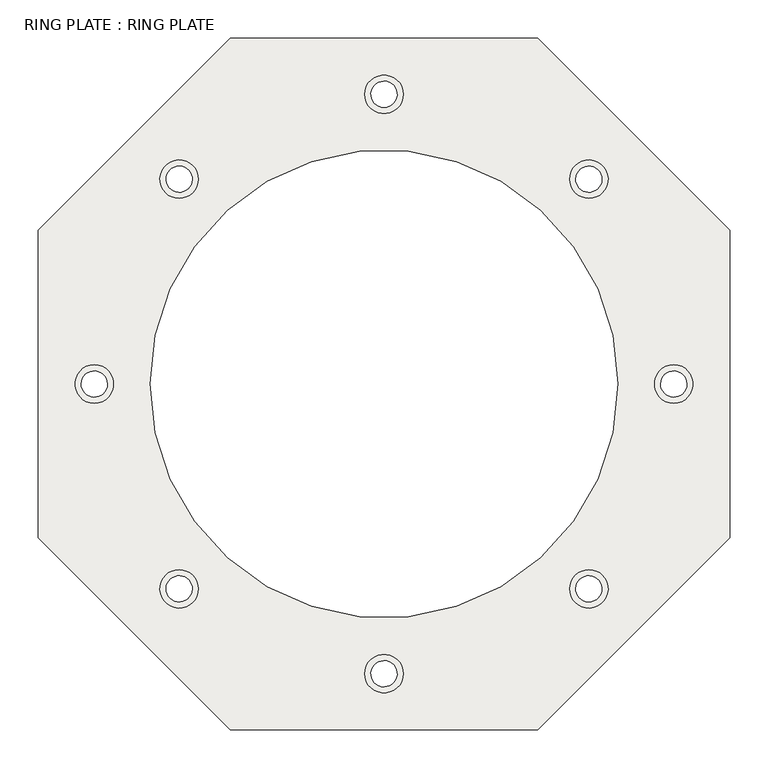
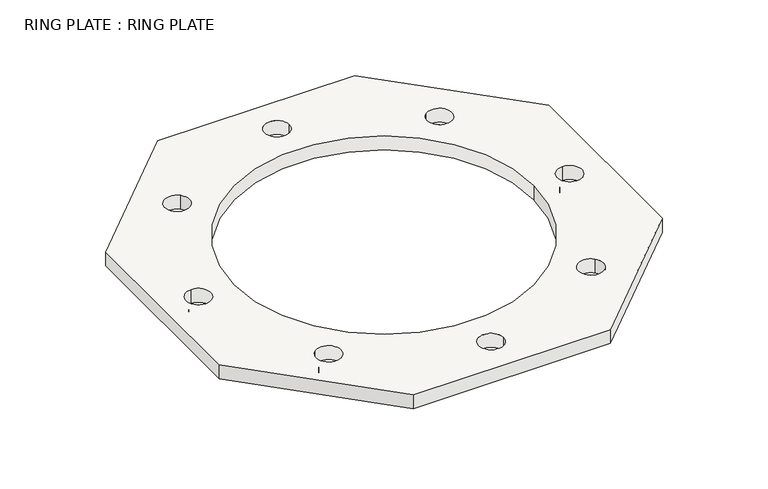
"""IFC4 building model written with IfcOpenShell, lengths in millimetres: slab geometry, RING PLATE : RING PLATE."""

from ifc_helpers import new_model, si_unit, point, frame, frame_2d, origin, place, context, project, spatial, polyline, circle_curve, trimmed, segment, composite_curve, outline, extrude, source, transform, mapped, element, save


def ring_plate_ring_plate_2bacfa3f(model_context):
    return source(origin(), model_context, "Body", "SweptSolid", [
        extrude(outline(polyline([(266.7560332, 19296.404436), (298.5758384, 19264.5846308), (316.2535079, 19246.9069613), (330.3956435, 19232.7648257), (266.7560332, 19169.1252154), (252.6138976, 19183.267351), (234.936228, 19200.9450205), (203.1164229, 19232.7648257), (266.7560332, 19296.404436)]), holes=[composite_curve([segment(trimmed(circle_curve(frame_2d((266.7560332, 19232.7648257)), 17.0), [point((266.1315996, 19215.7762977))], [point((267.3804668, 19249.7533537))], True, "CARTESIAN"), True, "CONTINUOUS"), segment(trimmed(circle_curve(frame_2d((266.7560332, 19232.7648257)), 17.0), [point((267.3804668, 19249.7533537))], [point((266.1315996, 19215.7762977))], True, "CARTESIAN"), True, "CONTINUOUS")], self_intersect=False)]), frame((0.0, 0.0, 200.0), z_axis=(0.0, 0.0, 1.0), x_axis=(1.0, 0.0, 0.0)), (0.0, 0.0, 1.0), 10.0),
        extrude(outline(polyline([(332.25, 19544.5208589), (377.25, 19544.5208589), (402.25, 19544.5208589), (422.25, 19544.5208589), (422.25, 19454.5208589), (402.25, 19454.5208589), (377.25, 19454.5208589), (332.25, 19454.5208589), (332.25, 19544.5208589)]), holes=[composite_curve([segment(trimmed(circle_curve(frame_2d((377.25, 19499.5208589)), 17.0), [point((388.8211621, 19487.0666143))], [point((365.6788379, 19511.9751035))], True, "CARTESIAN"), True, "CONTINUOUS"), segment(trimmed(circle_curve(frame_2d((377.25, 19499.5208589)), 17.0), [point((365.6788379, 19511.9751035))], [point((388.8211621, 19487.0666143))], True, "CARTESIAN"), True, "CONTINUOUS")], self_intersect=False)]), frame((0.0, 0.0, 200.0), z_axis=(0.0, 0.0, 1.0), x_axis=(1.0, 0.0, 0.0)), (0.0, 0.0, 1.0), 10.0),
        extrude(outline(polyline([(203.1164229, 19766.2768921), (234.936228, 19798.0966972), (252.6138976, 19815.7743668), (266.7560332, 19829.9165024), (330.3956435, 19766.2768921), (316.2535079, 19752.1347565), (298.5758384, 19734.4570869), (266.7560332, 19702.6372818), (203.1164229, 19766.2768921)]), holes=[composite_curve([segment(trimmed(circle_curve(frame_2d((266.7560332, 19766.2768921)), 17.0), [point((283.7445612, 19765.6524585))], [point((249.7675052, 19766.9013257))], True, "CARTESIAN"), True, "CONTINUOUS"), segment(trimmed(circle_curve(frame_2d((266.7560332, 19766.2768921)), 17.0), [point((249.7675052, 19766.9013257))], [point((283.7445612, 19765.6524585))], True, "CARTESIAN"), True, "CONTINUOUS")], self_intersect=False)]), frame((0.0, 0.0, 200.0), z_axis=(0.0, 0.0, 1.0), x_axis=(1.0, 0.0, 0.0)), (0.0, 0.0, 1.0), 10.0),
        extrude(outline(polyline([(-45.0, 19831.7708589), (-45.0, 19876.7708589), (-45.0, 19901.7708589), (-45.0, 19921.7708589), (45.0, 19921.7708589), (45.0, 19901.7708589), (45.0, 19876.7708589), (45.0, 19831.7708589), (-45.0, 19831.7708589)]), holes=[composite_curve([segment(trimmed(circle_curve(frame_2d((0.0, 19876.7708589)), 17.0), [point((12.4542446, 19888.342021))], [point((-12.4542446, 19865.1996968))], True, "CARTESIAN"), True, "CONTINUOUS"), segment(trimmed(circle_curve(frame_2d((0.0, 19876.7708589)), 17.0), [point((-12.4542446, 19865.1996968))], [point((12.4542446, 19888.342021))], True, "CARTESIAN"), True, "CONTINUOUS")], self_intersect=False)]), frame((0.0, 0.0, 200.0), z_axis=(0.0, 0.0, 1.0), x_axis=(1.0, 0.0, 0.0)), (0.0, 0.0, 1.0), 10.0),
        extrude(outline(polyline([(-266.7560332, 19702.6372818), (-298.5758384, 19734.4570869), (-316.2535079, 19752.1347565), (-330.3956435, 19766.2768921), (-266.7560332, 19829.9165024), (-252.6138976, 19815.7743668), (-234.936228, 19798.0966972), (-203.1164229, 19766.2768921), (-266.7560332, 19702.6372818)]), holes=[composite_curve([segment(trimmed(circle_curve(frame_2d((-266.7560332, 19766.2768921)), 17.0), [point((-266.1315996, 19783.2654201))], [point((-267.3804668, 19749.2883641))], True, "CARTESIAN"), True, "CONTINUOUS"), segment(trimmed(circle_curve(frame_2d((-266.7560332, 19766.2768921)), 17.0), [point((-267.3804668, 19749.2883641))], [point((-266.1315996, 19783.2654201))], True, "CARTESIAN"), True, "CONTINUOUS")], self_intersect=False)]), frame((0.0, 0.0, 200.0), z_axis=(0.0, 0.0, 1.0), x_axis=(1.0, 0.0, 0.0)), (0.0, 0.0, 1.0), 10.0),
        extrude(outline(polyline([(-332.25, 19454.5208589), (-377.25, 19454.5208589), (-402.25, 19454.5208589), (-433.7911596, 19454.5208589), (-433.7911596, 19544.5208589), (-402.25, 19544.5208589), (-377.25, 19544.5208589), (-332.25, 19544.5208589), (-332.25, 19454.5208589)]), holes=[composite_curve([segment(trimmed(circle_curve(frame_2d((-377.25, 19499.5208589)), 17.0), [point((-388.8211621, 19511.9751035))], [point((-365.6788379, 19487.0666143))], True, "CARTESIAN"), True, "CONTINUOUS"), segment(trimmed(circle_curve(frame_2d((-377.25, 19499.5208589)), 17.0), [point((-365.6788379, 19487.0666143))], [point((-388.8211621, 19511.9751035))], True, "CARTESIAN"), True, "CONTINUOUS")], self_intersect=False)]), frame((0.0, 0.0, 200.0), z_axis=(0.0, 0.0, 1.0), x_axis=(1.0, 0.0, 0.0)), (0.0, 0.0, 1.0), 10.0),
        extrude(outline(polyline([(-203.1164229, 19232.7648257), (-234.936228, 19200.9450205), (-252.6138976, 19183.267351), (-266.7560332, 19169.1252154), (-330.3956435, 19232.7648257), (-316.2535079, 19246.9069613), (-298.5758384, 19264.5846308), (-266.7560332, 19296.404436), (-203.1164229, 19232.7648257)]), holes=[composite_curve([segment(trimmed(circle_curve(frame_2d((-266.7560332, 19232.7648257)), 17.0), [point((-283.7445612, 19233.3892593))], [point((-249.7675052, 19232.1403921))], True, "CARTESIAN"), True, "CONTINUOUS"), segment(trimmed(circle_curve(frame_2d((-266.7560332, 19232.7648257)), 17.0), [point((-249.7675052, 19232.1403921))], [point((-283.7445612, 19233.3892593))], True, "CARTESIAN"), True, "CONTINUOUS")], self_intersect=False)]), frame((0.0, 0.0, 200.0), z_axis=(0.0, 0.0, 1.0), x_axis=(1.0, 0.0, 0.0)), (0.0, 0.0, 1.0), 10.0),
        extrude(outline(polyline([(45.0, 19167.2708589), (45.0, 19122.2708589), (45.0, 19097.2708589), (45.0, 19077.2708589), (-45.0, 19077.2708589), (-45.0, 19097.2708589), (-45.0, 19122.2708589), (-45.0, 19167.2708589), (45.0, 19167.2708589)]), holes=[composite_curve([segment(trimmed(circle_curve(frame_2d((0.0, 19122.2708589)), 17.0), [point((-12.4542446, 19110.6996968))], [point((12.4542446, 19133.842021))], True, "CARTESIAN"), True, "CONTINUOUS"), segment(trimmed(circle_curve(frame_2d((0.0, 19122.2708589)), 17.0), [point((12.4542446, 19133.842021))], [point((-12.4542446, 19110.6996968))], True, "CARTESIAN"), True, "CONTINUOUS")], self_intersect=False)]), frame((0.0, 0.0, 200.0), z_axis=(0.0, 0.0, 1.0), x_axis=(1.0, 0.0, 0.0)), (0.0, 0.0, 1.0), 10.0),
        extrude(outline(polyline([(-450.0, 19699.5208589), (-200.0, 19949.5208589), (200.0, 19949.5208589), (450.0, 19699.5208589), (450.0, 19299.5208589), (200.0, 19049.5208589), (-200.0, 19049.5208589), (-450.0, 19299.5208589), (-450.0, 19699.5208589)]), holes=[composite_curve([segment(trimmed(circle_curve(frame_2d((0.0, 19499.5208589)), 304.5), [point((-304.5, 19499.5208589))], [point((304.5, 19499.5208589))], True, "CARTESIAN"), True, "CONTINUOUS"), segment(trimmed(circle_curve(frame_2d((0.0, 19499.5208589)), 304.5), [point((304.5, 19499.5208589))], [point((-304.5, 19499.5208589))], True, "CARTESIAN"), True, "CONTINUOUS")], self_intersect=False), composite_curve([segment(trimmed(circle_curve(frame_2d((0.0, 19122.2708589)), 25.0), [point((-25.0, 19122.2708589))], [point((25.0, 19122.2708589))], True, "CARTESIAN"), True, "CONTINUOUS"), segment(trimmed(circle_curve(frame_2d((0.0, 19122.2708589)), 25.0), [point((25.0, 19122.2708589))], [point((-25.0, 19122.2708589))], True, "CARTESIAN"), True, "CONTINUOUS")], self_intersect=False), composite_curve([segment(trimmed(circle_curve(frame_2d((-266.7560332, 19232.7648257)), 25.0), [point((-284.4337027, 19250.4424952))], [point((-249.0783637, 19215.0871562))], True, "CARTESIAN"), True, "CONTINUOUS"), segment(trimmed(circle_curve(frame_2d((-266.7560332, 19232.7648257)), 25.0), [point((-249.0783637, 19215.0871562))], [point((-284.4337027, 19250.4424952))], True, "CARTESIAN"), True, "CONTINUOUS")], self_intersect=False), composite_curve([segment(trimmed(circle_curve(frame_2d((-377.25, 19499.5208589)), 25.0), [point((-377.25, 19524.5208589))], [point((-377.25, 19474.5208589))], True, "CARTESIAN"), True, "CONTINUOUS"), segment(trimmed(circle_curve(frame_2d((-377.25, 19499.5208589)), 25.0), [point((-377.25, 19474.5208589))], [point((-377.25, 19524.5208589))], True, "CARTESIAN"), True, "CONTINUOUS")], self_intersect=False), composite_curve([segment(trimmed(circle_curve(frame_2d((-266.7560332, 19766.2768921)), 25.0), [point((-249.0783637, 19783.9545616))], [point((-284.4337027, 19748.5992226))], True, "CARTESIAN"), True, "CONTINUOUS"), segment(trimmed(circle_curve(frame_2d((-266.7560332, 19766.2768921)), 25.0), [point((-284.4337027, 19748.5992226))], [point((-249.0783637, 19783.9545616))], True, "CARTESIAN"), True, "CONTINUOUS")], self_intersect=False), composite_curve([segment(trimmed(circle_curve(frame_2d((0.0, 19876.7708589)), 25.0), [point((25.0, 19876.7708589))], [point((-25.0, 19876.7708589))], True, "CARTESIAN"), True, "CONTINUOUS"), segment(trimmed(circle_curve(frame_2d((0.0, 19876.7708589)), 25.0), [point((-25.0, 19876.7708589))], [point((25.0, 19876.7708589))], True, "CARTESIAN"), True, "CONTINUOUS")], self_intersect=False), composite_curve([segment(trimmed(circle_curve(frame_2d((266.7560332, 19766.2768921)), 25.0), [point((284.4337027, 19748.5992226))], [point((249.0783637, 19783.9545616))], True, "CARTESIAN"), True, "CONTINUOUS"), segment(trimmed(circle_curve(frame_2d((266.7560332, 19766.2768921)), 25.0), [point((249.0783637, 19783.9545616))], [point((284.4337027, 19748.5992226))], True, "CARTESIAN"), True, "CONTINUOUS")], self_intersect=False), composite_curve([segment(trimmed(circle_curve(frame_2d((377.25, 19499.5208589)), 25.0), [point((377.25, 19474.5208589))], [point((377.25, 19524.5208589))], True, "CARTESIAN"), True, "CONTINUOUS"), segment(trimmed(circle_curve(frame_2d((377.25, 19499.5208589)), 25.0), [point((377.25, 19524.5208589))], [point((377.25, 19474.5208589))], True, "CARTESIAN"), True, "CONTINUOUS")], self_intersect=False), composite_curve([segment(trimmed(circle_curve(frame_2d((266.7560332, 19232.7648257)), 25.0), [point((249.0783637, 19215.0871562))], [point((284.4337027, 19250.4424952))], True, "CARTESIAN"), True, "CONTINUOUS"), segment(trimmed(circle_curve(frame_2d((266.7560332, 19232.7648257)), 25.0), [point((284.4337027, 19250.4424952))], [point((249.0783637, 19215.0871562))], True, "CARTESIAN"), True, "CONTINUOUS")], self_intersect=False)]), frame((0.0, 0.0, 210.0), z_axis=(0.0, 0.0, 1.0), x_axis=(1.0, 0.0, 0.0)), (0.0, 0.0, 1.0), 30.0),
    ])


if __name__ == "__main__":
    model = new_model("IFC4")
    model_context = context("Model", 3, world=origin())
    ifc_project = project(units=[si_unit("LENGTHUNIT", "METRE", prefix="MILLI")], contexts=[model_context])
    site = spatial("IfcSite", under=ifc_project)
    building = spatial("IfcBuilding", under=site)
    placement = place(None, origin())
    ring_plate_ring_plate_shape = ring_plate_ring_plate_2bacfa3f(model_context)
    element("IfcSlab", 1, ObjectType="RING PLATE : RING PLATE", at=placement, inside=building, context=model_context, shape_type="MappedRepresentation", body=[
        mapped(ring_plate_ring_plate_shape, transform((0.0, 0.0, 0.0), x_axis=(1.0, 0.0, 0.0), y_axis=(0.0, 1.0, 0.0), z_axis=(0.0, 0.0, 1.0))),
    ])
    save(model, "model.ifc")
